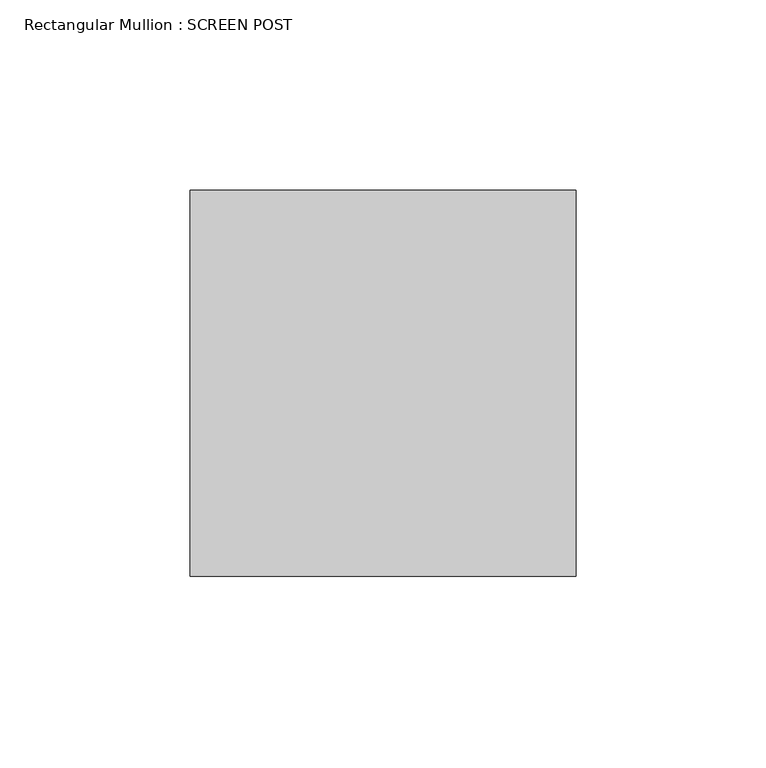
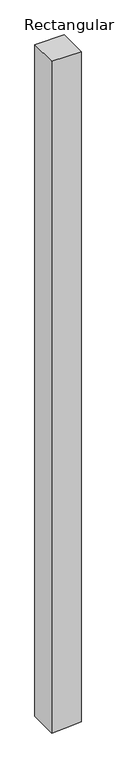
"""IFC4 building model written with IfcOpenShell, lengths in millimetres: member geometry, Rectangular Mullion : SCREEN POST."""

from ifc_helpers import new_model, si_unit, frame, origin, place, context, project, spatial, polyline, outline, extrude, source, transform, mapped, element, save


def rectangular_mullion_screen_post_ae30e3d1(model_context):
    return source(origin(), model_context, "Body", "SweptSolid", [
        extrude(outline(polyline([(0.0, 50.8), (0.0, -50.8), (-2466.4714509, -50.8), (-2463.692553, -6.3376339), (-2460.1214509, 50.8), (0.0, 50.8)])), frame((0.0, -50.8, 0.0), z_axis=(0.0, 1.0, 0.0), x_axis=(0.0, 0.0, 1.0)), (0.0, 0.0, 1.0), 101.6),
    ])


if __name__ == "__main__":
    model = new_model("IFC4")
    model_context = context("Model", 3, world=origin())
    ifc_project = project(units=[si_unit("LENGTHUNIT", "METRE", prefix="MILLI")], contexts=[model_context])
    site = spatial("IfcSite", under=ifc_project)
    building = spatial("IfcBuilding", under=site)
    placement = place(None, origin())
    rectangular_mullion_screen_post_shape = rectangular_mullion_screen_post_ae30e3d1(model_context)
    element("IfcMember", 1, ObjectType="Rectangular Mullion : SCREEN POST", at=placement, inside=building, context=model_context, shape_type="MappedRepresentation", body=[
        mapped(rectangular_mullion_screen_post_shape, transform((0.0, 0.0, 0.0), x_axis=(1.0, 0.0, 0.0), y_axis=(0.0, 1.0, 0.0), z_axis=(0.0, 0.0, 1.0))),
    ])
    save(model, "model.ifc")

# Revit data of these elements
# Type "Rectangular Mullion : SCREEN POST"
#   built-in parameter 1007304 = 0.333333 (stored number, unit not read)
#   built-in parameter 1007301 = 0.166667 (stored number, unit not read)
#   built-in parameter 1007300 = 0.166667 (stored number, unit not read)
# Element 1 (IfcMember, "Rectangular Mullion : SCREEN POST")
#   Materials on its faces: "GLULAMS COLUMNS\n(PRESSURE TREATED W/ PENTA IN SOLVENT) (EXTERIOR STAIN: PENOFIN VERDE EXT. STAIN - COLOR: CEDAR)"
# Materials
#   "GLULAMS COLUMNS\n(PRESSURE TREATED W/ PENTA IN SOLVENT) (EXTERIOR STAIN: PENOFIN VERDE EXT. STAIN - COLOR: CEDAR)": class "Wood", colour RGB 164 134 123, transparency 0, Description = "Pinus Echinata", Cost = 0
